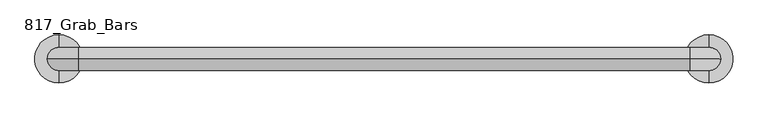
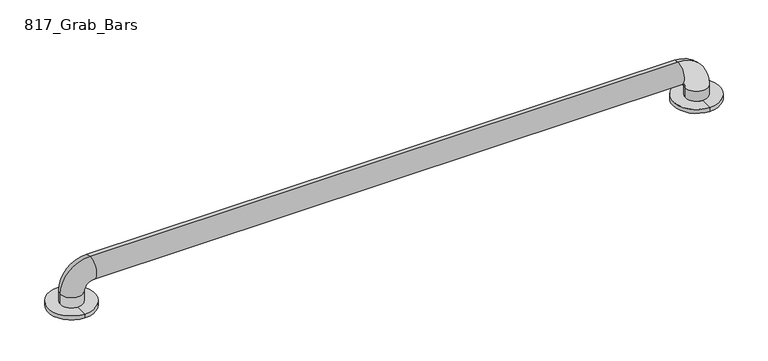
"""IFC4 building model written with IfcOpenShell, lengths in millimetres: proxy geometry, 817_Grab_Bars : 8170-001420."""

from ifc_helpers import new_model, si_unit, point, frame, origin, place, context, project, spatial, circle_curve, ellipse_curve, trimmed, source, transform, mapped, element, save
from ifc_brep_helpers import plane_surface, cylinder_surface, revolved_surface, advanced_brep


def proxy_817_grab_bars_30642a4a(model_context):
    return source(origin(), model_context, "Body", "AdvancedBrep", [
        advanced_brep(
        [(-439.7375, 496.8875, 7.14375), (-439.7375, 517.525, 7.14375), (-458.7875, 536.575, 7.14375), (-439.7375, 555.625, 7.14375), (-439.7375, 576.2625, 7.14375), (-420.6875, 536.575, 7.14375), (-439.7375, 576.2625, 0.0), (-439.7375, 555.625, 0.0), (-439.7375, 536.575, 0.0), (-439.7375, 517.525, 0.0), (-439.7375, 496.8875, 0.0), (627.0625, 496.8875, 7.14375), (627.0625, 517.525, 7.14375), (608.0125, 536.575, 7.14375), (627.0625, 555.625, 7.14375), (627.0625, 576.2625, 7.14375), (646.1125, 536.575, 7.14375), (627.0625, 576.2625, 0.0), (627.0625, 555.625, 0.0), (627.0625, 536.575, 0.0), (627.0625, 517.525, 0.0), (627.0625, 496.8875, 0.0), (-458.7875, 536.575, 25.4), (-420.6875, 536.575, 25.4), (-407.9875, 536.575, 38.1), (-407.9875, 536.575, 76.2), (595.3125, 536.575, 38.1), (595.3125, 536.575, 76.2), (608.0125, 536.575, 25.4), (646.1125, 536.575, 25.4)],
        [
            (0, 1),
            (1, 2, circle_curve(frame((-439.7375, 536.575, 7.14375), z_axis=(0.0, 0.0, -1.0), x_axis=(1.0, 0.0, 0.0)), 19.05)),
            (2, 3, circle_curve(frame((-439.7375, 536.575, 7.14375), z_axis=(0.0, 0.0, -1.0), x_axis=(1.0, 0.0, 0.0)), 19.05)),
            (3, 4),
            (4, 0, circle_curve(frame((-439.7375, 536.575, 7.14375), z_axis=(0.0, 0.0, 1.0), x_axis=(0.0, -1.0, 0.0)), 39.6875)),
            (3, 5, circle_curve(frame((-439.7375, 536.575, 7.14375), z_axis=(0.0, 0.0, -1.0), x_axis=(1.0, 0.0, 0.0)), 19.05)),
            (5, 1, circle_curve(frame((-439.7375, 536.575, 7.14375), z_axis=(0.0, 0.0, -1.0), x_axis=(1.0, 0.0, 0.0)), 19.05)),
            (0, 4, circle_curve(frame((-439.7375, 536.575, 7.14375), z_axis=(0.0, 0.0, 1.0), x_axis=(0.0, -1.0, 0.0)), 39.6875)),
            (6, 7),
            (7, 8),
            (8, 9),
            (9, 10),
            (10, 6, circle_curve(frame((-439.7375, 536.575, 0.0), z_axis=(0.0, 0.0, -1.0), x_axis=(0.0, -1.0, 0.0)), 39.6875)),
            (6, 10, circle_curve(frame((-439.7375, 536.575, 0.0), z_axis=(0.0, 0.0, -1.0), x_axis=(0.0, -1.0, 0.0)), 39.6875)),
            (4, 6),
            (10, 0),
            (11, 12),
            (12, 13, circle_curve(frame((627.0625, 536.575, 7.14375), z_axis=(0.0, 0.0, -1.0), x_axis=(-1.0, 0.0, 0.0)), 19.05)),
            (13, 14, circle_curve(frame((627.0625, 536.575, 7.14375), z_axis=(0.0, 0.0, -1.0), x_axis=(-1.0, 0.0, 0.0)), 19.05)),
            (14, 15),
            (15, 11, circle_curve(frame((627.0625, 536.575, 7.14375), z_axis=(0.0, 0.0, 1.0), x_axis=(0.0, -1.0, 0.0)), 39.6875)),
            (14, 16, circle_curve(frame((627.0625, 536.575, 7.14375), z_axis=(0.0, 0.0, -1.0), x_axis=(-1.0, 0.0, 0.0)), 19.05)),
            (16, 12, circle_curve(frame((627.0625, 536.575, 7.14375), z_axis=(0.0, 0.0, -1.0), x_axis=(-1.0, 0.0, 0.0)), 19.05)),
            (11, 15, circle_curve(frame((627.0625, 536.575, 7.14375), z_axis=(0.0, 0.0, 1.0), x_axis=(0.0, -1.0, 0.0)), 39.6875)),
            (17, 18),
            (18, 19),
            (19, 20),
            (20, 21),
            (21, 17, circle_curve(frame((627.0625, 536.575, 0.0), z_axis=(0.0, 0.0, -1.0), x_axis=(0.0, -1.0, 0.0)), 39.6875)),
            (17, 21, circle_curve(frame((627.0625, 536.575, 0.0), z_axis=(0.0, 0.0, -1.0), x_axis=(0.0, -1.0, 0.0)), 39.6875)),
            (15, 17),
            (21, 11),
            (22, 2),
            (5, 23),
            (23, 22, circle_curve(frame((-439.7375, 536.575, 25.4), z_axis=(0.0, 0.0, -1.0), x_axis=(1.0, 0.0, 0.0)), 19.05)),
            (22, 23, circle_curve(frame((-439.7375, 536.575, 25.4), z_axis=(0.0, 0.0, -1.0), x_axis=(1.0, 0.0, 0.0)), 19.05)),
            (23, 24, circle_curve(frame((-407.9875, 536.575, 25.4), z_axis=(0.0, 1.0, 0.0), x_axis=(-1.0, 0.0, 0.0)), 12.7)),
            (24, 25, circle_curve(frame((-407.9875, 536.575, 57.15), z_axis=(-1.0, 0.0, 0.0), x_axis=(0.0, 0.0, -1.0)), 19.05)),
            (25, 22, circle_curve(frame((-407.9875, 536.575, 25.4), z_axis=(0.0, -1.0, 0.0), x_axis=(-1.0, 0.0, 0.0)), 50.8)),
            (25, 24, circle_curve(frame((-407.9875, 536.575, 57.15), z_axis=(-1.0, 0.0, 0.0), x_axis=(0.0, 0.0, -1.0)), 19.05)),
            (24, 26),
            (26, 27, circle_curve(frame((595.3125, 536.575, 57.15), z_axis=(-1.0, 0.0, 0.0), x_axis=(0.0, 0.0, -1.0)), 19.05)),
            (27, 25),
            (27, 26, circle_curve(frame((595.3125, 536.575, 57.15), z_axis=(-1.0, 0.0, 0.0), x_axis=(0.0, 0.0, -1.0)), 19.05)),
            (26, 28, circle_curve(frame((595.3125, 536.575, 25.4), z_axis=(0.0, 1.0, 0.0), x_axis=(0.0, 0.0, 1.0)), 12.7)),
            (28, 29, circle_curve(frame((627.0625, 536.575, 25.4), z_axis=(0.0, 0.0, 1.0), x_axis=(-1.0, 0.0, 0.0)), 19.05)),
            (29, 27, circle_curve(frame((595.3125, 536.575, 25.4), z_axis=(0.0, -1.0, 0.0), x_axis=(0.0, 0.0, 1.0)), 50.8)),
            (29, 28, circle_curve(frame((627.0625, 536.575, 25.4), z_axis=(0.0, 0.0, 1.0), x_axis=(-1.0, 0.0, 0.0)), 19.05)),
            (28, 13),
            (16, 29),
        ],
        [
            plane_surface(frame((-439.7375, 536.575, 7.14375), z_axis=(0.0, 0.0, 1.0), x_axis=(0.0, -1.0, 0.0))),
            plane_surface(frame((-439.7375, 536.575, 0.0), z_axis=(0.0, 0.0, -1.0), x_axis=(0.0, -1.0, 0.0))),
            cylinder_surface(frame((-439.7375, 536.575, 7.14375), z_axis=(0.0, 0.0, 1.0), x_axis=(0.0, -1.0, 0.0)), 39.6875),
            plane_surface(frame((627.0625, 536.575, 7.14375), z_axis=(0.0, 0.0, 1.0), x_axis=(0.0, -1.0, 0.0))),
            plane_surface(frame((627.0625, 536.575, 0.0), z_axis=(0.0, 0.0, -1.0), x_axis=(0.0, -1.0, 0.0))),
            cylinder_surface(frame((627.0625, 536.575, 31.75), z_axis=(0.0, 0.0, 1.0), x_axis=(0.0, -1.0, 0.0)), 39.6875),
            cylinder_surface(frame((-439.7375, 536.575, 0.0), z_axis=(0.0, 0.0, -1.0), x_axis=(1.0, 0.0, 0.0)), 19.05),
            revolved_surface(trimmed(ellipse_curve(frame((-439.7375, 536.575, 25.4), z_axis=(0.0, 0.0, 1.0), x_axis=(1.0, 0.0, 0.0)), 19.05, 19.05), [point((-458.7875, 536.575, 25.4))], [point((-420.6875, 536.575, 25.4))], True, "CARTESIAN"), (-407.9875, 536.575, 25.4), (0.0, -1.0, 0.0)),
            revolved_surface(trimmed(ellipse_curve(frame((-439.7375, 536.575, 25.4), z_axis=(0.0, 0.0, 1.0), x_axis=(1.0, 0.0, 0.0)), 19.05, 19.05), [point((-420.6875, 536.575, 25.4))], [point((-458.7875, 536.575, 25.4))], True, "CARTESIAN"), (-407.9875, 536.575, 25.4), (0.0, -1.0, 0.0)),
            cylinder_surface(frame((-407.9875, 536.575, 57.15), z_axis=(-1.0, 0.0, 0.0), x_axis=(0.0, 0.0, -1.0)), 19.05),
            revolved_surface(trimmed(ellipse_curve(frame((595.3125, 536.575, 57.15), z_axis=(1.0, 0.0, 0.0), x_axis=(0.0, 0.0, -1.0)), 19.05, 19.05), [point((595.3125, 536.575, 76.2))], [point((595.3125, 536.575, 38.1))], True, "CARTESIAN"), (595.3125, 536.575, 25.4), (0.0, -1.0, 0.0)),
            revolved_surface(trimmed(ellipse_curve(frame((595.3125, 536.575, 57.15), z_axis=(1.0, 0.0, 0.0), x_axis=(0.0, 0.0, -1.0)), 19.05, 19.05), [point((595.3125, 536.575, 38.1))], [point((595.3125, 536.575, 76.2))], True, "CARTESIAN"), (595.3125, 536.575, 25.4), (0.0, -1.0, 0.0)),
            cylinder_surface(frame((627.0625, 536.575, 25.4), z_axis=(0.0, 0.0, 1.0), x_axis=(-1.0, 0.0, 0.0)), 19.05),
        ],
        [
            (0, [[1, 2, 3, 4, 5]]),
            (0, [[-4, 6, 7, -1, 8]]),
            (1, [[9, 10, 11, 12, 13]]),
            (1, [[-12, -11, -10, -9, 14]]),
            (2, [[15, -13, 16, -5]]),
            (2, [[-16, -14, -15, -8]]),
            (3, [[17, 18, 19, 20, 21]]),
            (3, [[-20, 22, 23, -17, 24]]),
            (4, [[25, 26, 27, 28, 29]]),
            (4, [[-28, -27, -26, -25, 30]]),
            (5, [[31, -29, 32, -21]]),
            (5, [[-32, -30, -31, -24]]),
            (6, [[33, -2, -7, 34, 35]]),
            (6, [[-34, -6, -3, -33, 36]]),
            (7, [[37, 38, 39, -35]]),
            (8, [[-39, 40, -37, -36]]),
            (9, [[41, 42, 43, -38]]),
            (9, [[-43, 44, -41, -40]]),
            (10, [[45, 46, 47, -42]]),
            (11, [[-47, 48, -45, -44]]),
            (12, [[49, -18, -23, 50, -46]]),
            (12, [[-50, -22, -19, -49, -48]]),
        ],
    ),
    ])


if __name__ == "__main__":
    model = new_model("IFC4")
    model_context = context("Model", 3, world=origin())
    ifc_project = project(units=[si_unit("LENGTHUNIT", "METRE", prefix="MILLI")], contexts=[model_context])
    site = spatial("IfcSite", under=ifc_project)
    building = spatial("IfcBuilding", under=site)
    placement = place(None, origin())
    proxy_817_grab_bars_shape = proxy_817_grab_bars_30642a4a(model_context)
    element("IfcBuildingElementProxy", 1, Name="817_Grab_Bars : 8170-001420", ObjectType="817_Grab_Bars : 8170-001420", at=placement, inside=building, context=model_context, shape_type="MappedRepresentation", body=[
        mapped(proxy_817_grab_bars_shape, transform((0.0, 0.0, 0.0), x_axis=(1.0, 0.0, 0.0), y_axis=(0.0, 1.0, 0.0), z_axis=(0.0, 0.0, 1.0))),
    ])
    save(model, "model.ifc")

# Revit data of these elements
# Type "817_Grab_Bars : 8170-001420"
#   Keynote = "M10281313.01"
#   Warranty Information = "Complete unit, one (1) year"
#   Version = "1.0"
#   Technical Data = "http://www.bradleycorp.com/products/techdata/8815.pdf"
#   URL = "www.bradleycorp.com"
#   Type Comments = "All grab bar configurations are specified using centerline to centerline dimensions."
#   OmniClass Title = ""
#   Modeling Code = ""
#   Model = "8170-001420"
#   Material Note = "FLANGES - 11 GA., TUBING - 18 GA."
#   MasterFormat Section Title = ""
#   Manufacturer = "Bradley Corporation"
#   LEED Credit = ""
#   Instructions [instance default] = "This is a face mounted fixture."
#   Industry Standards = "ANSI Standard A117.1, ADA, ABA, ADAAG, UFAS"
#   Fire Rating = "None"
#   Description = "Grab Bars"
#   Copyright = "This Model Data is Property of Bradley Corporation"
#   Complies to NAFTA = "Yes"
#   Complies To Buy American Act = "Yes"
#   Assembly Code = "C1030200"
#   ADA Compliant = "Yes"
#   Radius = 0' - 0 3/4"
#   Percentage of Recycled Content = 56.77
#   Overall Length = 3' - 9 1/8"
#   OmniClass Number = 0
#   MasterFormat Section Number = 0
#   Length = 3' - 6"
#   Diameter = 0' - 1 1/2"
#   Default Elevation = 2' - 9"
#   Material and Finish = Bradley Corp Stainless Steel - Satin
# Element 1 (IfcBuildingElementProxy, "817_Grab_Bars : 8170-001420")
#   Materials on its faces: "Bradley Corp Stainless Steel - Satin"
# Materials
#   "Bradley Corp Stainless Steel - Satin": class "Metal", colour RGB 189 187 185, transparency 0, Manufacturer = "Bradley Corporation", URL = "www.bradleycorp.com", Description = "Stainless Steel - Satin Finish", Cost = 0
